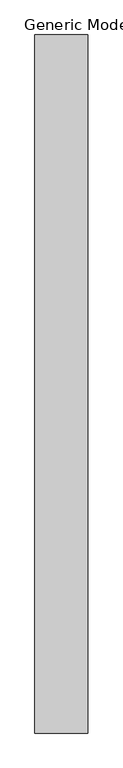
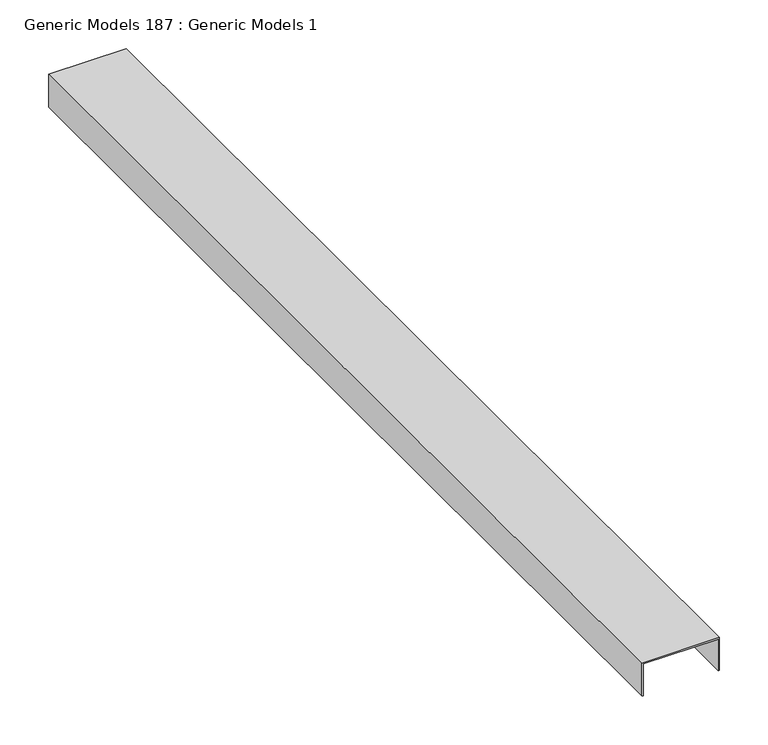
"""IFC4 building model written with IfcOpenShell, lengths in millimetres: proxy geometry, Generic Models 187 : Generic Models 1."""

from ifc_helpers import new_model, si_unit, frame, origin, place, context, project, spatial, polyline, outline, extrude, source, transform, mapped, element, save


def generic_models_187_generic_models_1_d2f1e0fb(model_context):
    return source(origin(), model_context, "Body", "SweptSolid", [
        extrude(outline(polyline([(2457.45, 49784.0), (2457.45, 49691.925), (2416.175, 49691.925), (2416.175, 49693.5125), (2455.8625, 49693.5125), (2455.8625, 49782.4125), (2416.175, 49782.4125), (2416.175, 49784.0), (2457.45, 49784.0)])), frame((0.0, 0.0, 0.0), z_axis=(0.0, 1.0, 0.0), x_axis=(0.0, 0.0, 1.0)), (0.0, 0.0, 1.0), 1219.2),
    ])


if __name__ == "__main__":
    model = new_model("IFC4")
    model_context = context("Model", 3, world=origin())
    ifc_project = project(units=[si_unit("LENGTHUNIT", "METRE", prefix="MILLI")], contexts=[model_context])
    site = spatial("IfcSite", under=ifc_project)
    building = spatial("IfcBuilding", under=site)
    placement = place(None, origin())
    generic_models_187_generic_models_1_shape = generic_models_187_generic_models_1_d2f1e0fb(model_context)
    element("IfcBuildingElementProxy", 1, Name="Generic Models 187 : Generic Models 1", ObjectType="Generic Models 187 : Generic Models 1", at=placement, inside=building, context=model_context, shape_type="MappedRepresentation", body=[
        mapped(generic_models_187_generic_models_1_shape, transform((0.0, 0.0, 0.0), x_axis=(1.0, 0.0, 0.0), y_axis=(0.0, 1.0, 0.0), z_axis=(0.0, 0.0, 1.0))),
    ])
    save(model, "model.ifc")

# Revit data of these elements
# Element 1 (IfcBuildingElementProxy, "Generic Models 187 : Generic Models 1")
#   Materials on its faces: "DEEP LEG OF DEFLECTION TRACK (2\" MIN. DEFLECTION)"
# Materials
#   "DEEP LEG OF DEFLECTION TRACK (2\" MIN. DEFLECTION)": class "Unassigned", colour RGB 210 209 208, transparency 0, Keynote = "M05121300.02", Cost = 0
